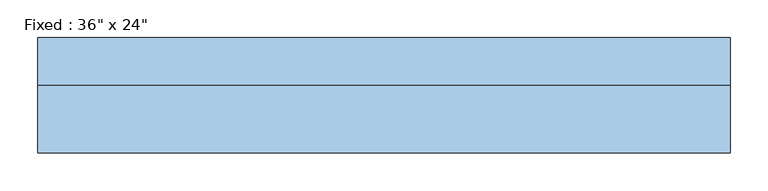
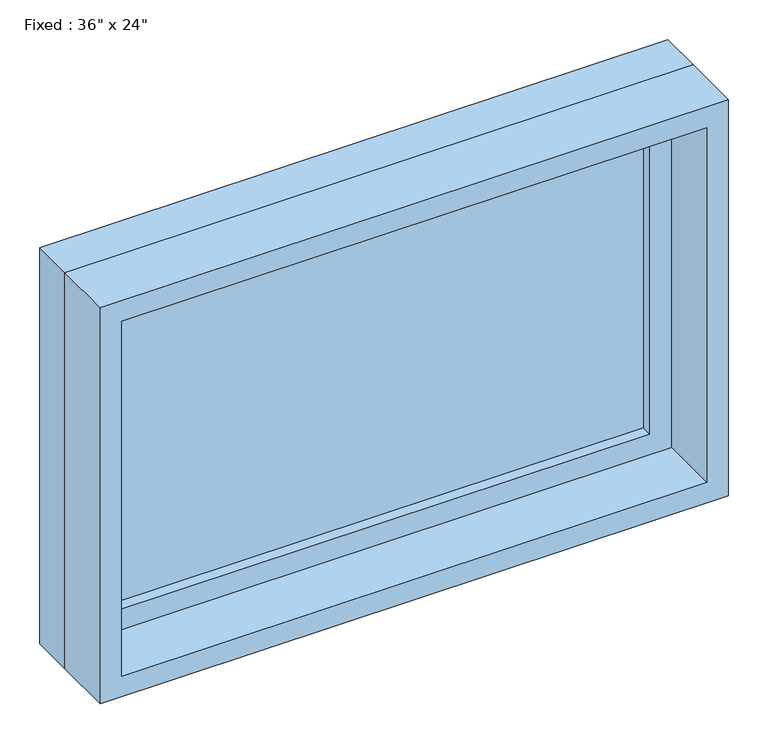
"""IFC4 building model written with IfcOpenShell, lengths in millimetres: window geometry."""

import ifcopenshell
import ifcopenshell.guid

model = None  # the IFC model being written
_history = None  # IfcOwnerHistory: only IFC2X3 demands one
_inside = {}  # id of a spatial element -> (the spatial element, [elements in it])
_under = {}  # id of a project, library or spatial element -> (it, [spatial elements below it])
_declared = {}  # id of a project -> (the project, [libraries it declares])
_typed = {}  # id of a type object -> (the type object, [elements of that type])
_made_of = {}  # id of a material, layer set ... -> (it, [elements and type objects made of it])


def new_model(schema):
    """Start an empty IFC model of exactly this schema.

    Asked for "IFC4X3", IfcOpenShell would pick the latest addendum, in which some entities
    have other attributes; the version numbers below select the first issue.
    IFC2X3 requires an IfcOwnerHistory on every rooted entity: one is made here for all.
    """
    global model, _history
    if schema == "IFC4X3":
        model = ifcopenshell.file(schema_version=(4, 3, 0, 0))
    else:
        model = ifcopenshell.file(schema=schema)
    _inside.clear()
    _under.clear()
    _declared.clear()
    _typed.clear()
    _made_of.clear()
    _history = None
    if model.schema == "IFC2X3":
        org = make("IfcOrganization", Name="unknown")
        user = make(
            "IfcPersonAndOrganization",
            ThePerson=make("IfcPerson", FamilyName="unknown"),
            TheOrganization=org,
        )
        app = make(
            "IfcApplication",
            ApplicationDeveloper=org,
            Version="unknown",
            ApplicationFullName="unknown",
            ApplicationIdentifier="unknown",
        )
        _history = make(
            "IfcOwnerHistory",
            OwningUser=user,
            OwningApplication=app,
            ChangeAction="ADDED",
            CreationDate=0,
        )
    return model


def make(cls, **values):
    """One entity of the class cls with the attributes given. An attribute that is None is left unset."""
    return model.create_entity(
        cls, **{name: value for name, value in values.items() if value is not None}
    )


def rooted(cls, **values):
    """An entity with a GlobalId (a new one), such as an element, a storey or a relation."""
    return make(cls, GlobalId=ifcopenshell.guid.new(), OwnerHistory=_history, **values)


def si_unit(unit_type, name, prefix=None):
    """IfcSIUnit, for example si_unit("LENGTHUNIT", "METRE", prefix="MILLI")."""
    return make("IfcSIUnit", UnitType=unit_type, Prefix=prefix, Name=name)


def assignment(units):
    """IfcUnitAssignment: the units of a project."""
    return None if units is None else make("IfcUnitAssignment", Units=units)


def point(xyz):
    """IfcCartesianPoint."""
    return None if xyz is None else make("IfcCartesianPoint", Coordinates=xyz)


def direction(xyz):
    """IfcDirection."""
    return None if xyz is None else make("IfcDirection", DirectionRatios=xyz)


def frame(location, z_axis=None, x_axis=None):
    """IfcAxis2Placement3D, a coordinate frame: its origin and axes. An axis left out is left unset."""
    return make(
        "IfcAxis2Placement3D",
        Location=point(location),
        Axis=direction(z_axis),
        RefDirection=direction(x_axis),
    )


def origin():
    """The frame at (0, 0, 0) with its axes left unset."""
    return frame((0.0, 0.0, 0.0))


def place(relative_to, where):
    """IfcLocalPlacement: puts the frame where relative to a parent placement (None: the world)."""
    return make(
        "IfcLocalPlacement", PlacementRelTo=relative_to, RelativePlacement=where
    )


def context(
    kind, dimensions, precision=None, world=None, true_north=None, identifier=None
):
    """IfcGeometricRepresentationContext, for example the 3D "Model" context."""
    return make(
        "IfcGeometricRepresentationContext",
        ContextIdentifier=identifier,
        ContextType=kind,
        CoordinateSpaceDimension=dimensions,
        Precision=precision,
        WorldCoordinateSystem=world,
        TrueNorth=true_north,
    )


def project(units=None, contexts=None):
    """IfcProject with its units and contexts."""
    return rooted(
        "IfcProject",
        Name="project",
        RepresentationContexts=contexts,
        UnitsInContext=assignment(units),
    )


def spatial(cls, under=None, at=None, **own):
    """A site, building, storey or space (cls), placed at a placement, below another one or the project."""
    s = rooted(cls, ObjectPlacement=at, **own)
    if under is not None:
        _under.setdefault(under.id(), (under, []))[1].append(s)
    return s


def polyline(points):
    """IfcPolyline through the points."""
    return make("IfcPolyline", Points=[point(p) for p in points])


def outline(outer, holes=None, kind="AREA"):
    """IfcArbitraryClosedProfileDef: a profile drawn as a closed curve; with holes, ...WithVoids."""
    if holes is None:
        return make("IfcArbitraryClosedProfileDef", ProfileType=kind, OuterCurve=outer)
    return make(
        "IfcArbitraryProfileDefWithVoids",
        ProfileType=kind,
        OuterCurve=outer,
        InnerCurves=holes,
    )


def extrude(swept, where, along, depth):
    """IfcExtrudedAreaSolid: the profile swept, set in the frame where, extruded along a direction by depth."""
    return make(
        "IfcExtrudedAreaSolid",
        SweptArea=swept,
        Position=where,
        ExtrudedDirection=direction(along),
        Depth=depth,
    )


def shape(context_of_items, identifier, shape_type, items):
    """IfcShapeRepresentation: the items that make up one representation, for example the "Body"."""
    return make(
        "IfcShapeRepresentation",
        ContextOfItems=context_of_items,
        RepresentationIdentifier=identifier,
        RepresentationType=shape_type,
        Items=items,
    )


def source(mapping_origin, context_of_items, identifier, shape_type, items):
    """IfcRepresentationMap: a shape defined once, which mapped items show again and again."""
    return make(
        "IfcRepresentationMap",
        MappingOrigin=mapping_origin,
        MappedRepresentation=shape(context_of_items, identifier, shape_type, items),
    )


def transform(
    local_origin,
    x_axis=None,
    y_axis=None,
    z_axis=None,
    scale=None,
    scale2=None,
    scale3=None,
    uniform=True,
):
    """IfcCartesianTransformationOperator3D, or its non-uniform kind. x_axis, y_axis, z_axis: its Axis1, 2, 3."""
    if uniform:
        return make(
            "IfcCartesianTransformationOperator3D",
            Axis1=direction(x_axis),
            Axis2=direction(y_axis),
            LocalOrigin=point(local_origin),
            Scale=scale,
            Axis3=direction(z_axis),
        )
    return make(
        "IfcCartesianTransformationOperator3DnonUniform",
        Axis1=direction(x_axis),
        Axis2=direction(y_axis),
        LocalOrigin=point(local_origin),
        Scale=scale,
        Axis3=direction(z_axis),
        Scale2=scale2,
        Scale3=scale3,
    )


def mapped(mapping_source, mapping_target):
    """IfcMappedItem: shows the shape of a source again, moved by a transform."""
    return make(
        "IfcMappedItem", MappingSource=mapping_source, MappingTarget=mapping_target
    )


def made_of(thing, what):
    """Note that an element or type object is made of a material, layer set ...; save() writes the relation."""
    if what is not None:
        _made_of.setdefault(what.id(), (what, []))[1].append(thing)
    return thing


def element(
    cls,
    number,
    at=None,
    inside=None,
    cuts=None,
    type_object=None,
    material=None,
    context=None,
    identifier="Body",
    shape_type=None,
    held_by="IfcProductDefinitionShape",
    body=None,
    shapes=None,
    **own,
):
    """One element of the class cls, such as IfcWall. Its Tag is "e" and its number.

    at: its placement. inside: the storey or other place that contains it. cuts: it is an
    opening in that element (IfcRelVoidsElement). A single representation is given by context,
    identifier, shape_type and body (its items); several are given by shapes. held_by: the class
    of the entity that holds the representations. save() writes the other relations.
    """
    e = rooted(cls, Tag="e%d" % number, ObjectPlacement=at, **own)
    if body is not None:
        shapes = [shape(context, identifier, shape_type, body)]
    if shapes is not None:
        e.Representation = make(held_by, Representations=shapes)
    if inside is not None:
        _inside.setdefault(inside.id(), (inside, []))[1].append(e)
    if cuts is not None:
        rooted(
            "IfcRelVoidsElement", RelatingBuildingElement=cuts, RelatedOpeningElement=e
        )
    if type_object is not None:
        _typed.setdefault(type_object.id(), (type_object, []))[1].append(e)
    return made_of(e, material)


def aggregate(whole, parts):
    """IfcRelAggregates: a whole, such as a stair, and the parts it consists of."""
    return rooted("IfcRelAggregates", RelatingObject=whole, RelatedObjects=parts)


def save(model, path):
    """Write the relations noted so far, then the file.

    IfcRelAggregates (storeys below a building ...), IfcRelContainedInSpatialStructure (elements
    in a storey), IfcRelDefinesByType, IfcRelAssociatesMaterial and IfcRelDeclares: one each for
    every whole, place, type object, material and project.
    """
    for whole, parts in _under.values():
        aggregate(whole, parts)
    for where, things in _inside.values():
        rooted(
            "IfcRelContainedInSpatialStructure",
            RelatedElements=things,
            RelatingStructure=where,
        )
    for kind, things in _typed.values():
        rooted("IfcRelDefinesByType", RelatedObjects=things, RelatingType=kind)
    for what, things in _made_of.values():
        rooted("IfcRelAssociatesMaterial", RelatedObjects=things, RelatingMaterial=what)
    for by, libraries in _declared.values():
        rooted("IfcRelDeclares", RelatingContext=by, RelatedDefinitions=libraries)
    model.write(path)


def window_fef7ae9c(model_context):
    return source(origin(), model_context, "Body", "SweptSolid", [
        extrude(outline(polyline([(355.6, 28.575), (-431.8, 28.575), (-431.8, 41.275), (355.6, 41.275), (355.6, 28.575)])), frame((0.0, 0.0, 977.9), z_axis=(0.0, 0.0, 1.0), x_axis=(1.0, 0.0, 0.0)), (0.0, 0.0, 1.0), 482.6),
        extrude(outline(polyline([(1504.95, -476.25), (933.45, -476.25), (933.45, 400.05), (1504.95, 400.05), (1504.95, -476.25)]), holes=[polyline([(1460.5, -431.8), (1460.5, 355.6), (977.9, 355.6), (977.9, -431.8), (1460.5, -431.8)])]), frame((0.0, 12.7, 0.0), z_axis=(0.0, 1.0, 0.0), x_axis=(0.0, 0.0, 1.0)), (0.0, 0.0, 1.0), 44.45),
        extrude(outline(polyline([(1524.0, -495.3), (914.4, -495.3), (914.4, 419.1), (1524.0, 419.1), (1524.0, -495.3)]), holes=[polyline([(1492.25, -463.55), (1492.25, 387.35), (946.15, 387.35), (946.15, -463.55), (1492.25, -463.55)])]), frame((0.0, -76.2, 0.0), z_axis=(0.0, 1.0, 0.0), x_axis=(0.0, 0.0, 1.0)), (0.0, 0.0, 1.0), 88.9),
        extrude(outline(polyline([(1524.0, 419.1), (1524.0, -495.3), (914.4, -495.3), (914.4, 419.1), (1524.0, 419.1)]), holes=[polyline([(1504.95, 400.05), (933.45, 400.05), (933.45, -476.25), (1504.95, -476.25), (1504.95, 400.05)])]), frame((0.0, 12.7, 0.0), z_axis=(0.0, 1.0, 0.0), x_axis=(0.0, 0.0, 1.0)), (0.0, 0.0, 1.0), 63.5),
    ])


if __name__ == "__main__":
    model = new_model("IFC4")
    model_context = context("Model", 3, world=origin())
    ifc_project = project(units=[si_unit("LENGTHUNIT", "METRE", prefix="MILLI")], contexts=[model_context])
    site = spatial("IfcSite", under=ifc_project)
    building = spatial("IfcBuilding", under=site)
    placement = place(None, origin())
    window_shape = window_fef7ae9c(model_context)
    element("IfcWindow", 1, ObjectType="Fixed : 36\" x 24\"", at=placement, inside=building, context=model_context, shape_type="MappedRepresentation", body=[
        mapped(window_shape, transform((0.0, 0.0, 0.0), x_axis=(1.0, 0.0, 0.0), y_axis=(0.0, 1.0, 0.0), z_axis=(0.0, 0.0, 1.0))),
    ])
    save(model, "model.ifc")

# Revit data of these elements
# Type "Fixed : 36\" x 24\""
#   Type Mark = "8"
#   Assembly Code = "B2020100"
#   Height = 2' - 0"
#   Default Sill Height = 3' - 0"
#   Width = 3' - 0"
#   Window Inset = 0' - 0 3/4"
#   Glass Pane Material = Glass
#   Sash Material = Sash
#   Wall Closure = (empty or 0)
# Element 1 (IfcWindow, "Fixed : 36\" x 24\"")
#   Materials on its faces: "Sash", "Glass"
# Materials
#   "Glass": class "Glass", colour RGB 218 227 224, transparency 0.85, Description = "Soda Lime Glass", Cost = 0
#   "Sash": class "Wood", colour RGB 136 99 55, transparency 0
